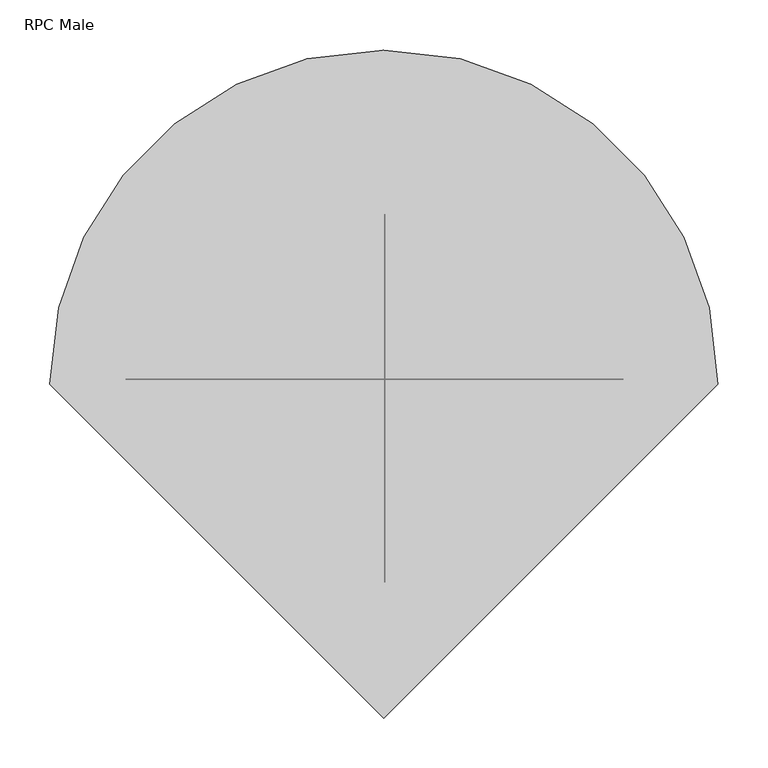
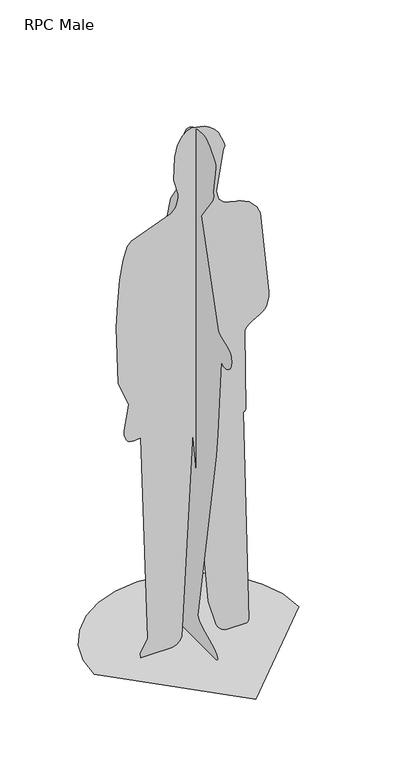
"""IFC4 building model written with IfcOpenShell, lengths in millimetres: proxy geometry, RPC Male : Dwayne."""

import ifcopenshell
import ifcopenshell.guid

model = None  # the IFC model being written
_history = None  # IfcOwnerHistory: only IFC2X3 demands one
_inside = {}  # id of a spatial element -> (the spatial element, [elements in it])
_under = {}  # id of a project, library or spatial element -> (it, [spatial elements below it])
_declared = {}  # id of a project -> (the project, [libraries it declares])
_typed = {}  # id of a type object -> (the type object, [elements of that type])
_made_of = {}  # id of a material, layer set ... -> (it, [elements and type objects made of it])


def new_model(schema):
    """Start an empty IFC model of exactly this schema.

    Asked for "IFC4X3", IfcOpenShell would pick the latest addendum, in which some entities
    have other attributes; the version numbers below select the first issue.
    IFC2X3 requires an IfcOwnerHistory on every rooted entity: one is made here for all.
    """
    global model, _history
    if schema == "IFC4X3":
        model = ifcopenshell.file(schema_version=(4, 3, 0, 0))
    else:
        model = ifcopenshell.file(schema=schema)
    _inside.clear()
    _under.clear()
    _declared.clear()
    _typed.clear()
    _made_of.clear()
    _history = None
    if model.schema == "IFC2X3":
        org = make("IfcOrganization", Name="unknown")
        user = make(
            "IfcPersonAndOrganization",
            ThePerson=make("IfcPerson", FamilyName="unknown"),
            TheOrganization=org,
        )
        app = make(
            "IfcApplication",
            ApplicationDeveloper=org,
            Version="unknown",
            ApplicationFullName="unknown",
            ApplicationIdentifier="unknown",
        )
        _history = make(
            "IfcOwnerHistory",
            OwningUser=user,
            OwningApplication=app,
            ChangeAction="ADDED",
            CreationDate=0,
        )
    return model


def make(cls, **values):
    """One entity of the class cls with the attributes given. An attribute that is None is left unset."""
    return model.create_entity(
        cls, **{name: value for name, value in values.items() if value is not None}
    )


def rooted(cls, **values):
    """An entity with a GlobalId (a new one), such as an element, a storey or a relation."""
    return make(cls, GlobalId=ifcopenshell.guid.new(), OwnerHistory=_history, **values)


def si_unit(unit_type, name, prefix=None):
    """IfcSIUnit, for example si_unit("LENGTHUNIT", "METRE", prefix="MILLI")."""
    return make("IfcSIUnit", UnitType=unit_type, Prefix=prefix, Name=name)


def assignment(units):
    """IfcUnitAssignment: the units of a project."""
    return None if units is None else make("IfcUnitAssignment", Units=units)


def point(xyz):
    """IfcCartesianPoint."""
    return None if xyz is None else make("IfcCartesianPoint", Coordinates=xyz)


def direction(xyz):
    """IfcDirection."""
    return None if xyz is None else make("IfcDirection", DirectionRatios=xyz)


def frame(location, z_axis=None, x_axis=None):
    """IfcAxis2Placement3D, a coordinate frame: its origin and axes. An axis left out is left unset."""
    return make(
        "IfcAxis2Placement3D",
        Location=point(location),
        Axis=direction(z_axis),
        RefDirection=direction(x_axis),
    )


def origin():
    """The frame at (0, 0, 0) with its axes left unset."""
    return frame((0.0, 0.0, 0.0))


def place(relative_to, where):
    """IfcLocalPlacement: puts the frame where relative to a parent placement (None: the world)."""
    return make(
        "IfcLocalPlacement", PlacementRelTo=relative_to, RelativePlacement=where
    )


def context(
    kind, dimensions, precision=None, world=None, true_north=None, identifier=None
):
    """IfcGeometricRepresentationContext, for example the 3D "Model" context."""
    return make(
        "IfcGeometricRepresentationContext",
        ContextIdentifier=identifier,
        ContextType=kind,
        CoordinateSpaceDimension=dimensions,
        Precision=precision,
        WorldCoordinateSystem=world,
        TrueNorth=true_north,
    )


def project(units=None, contexts=None):
    """IfcProject with its units and contexts."""
    return rooted(
        "IfcProject",
        Name="project",
        RepresentationContexts=contexts,
        UnitsInContext=assignment(units),
    )


def spatial(cls, under=None, at=None, **own):
    """A site, building, storey or space (cls), placed at a placement, below another one or the project."""
    s = rooted(cls, ObjectPlacement=at, **own)
    if under is not None:
        _under.setdefault(under.id(), (under, []))[1].append(s)
    return s


def point_list(points):
    """IfcCartesianPointList2D or 3D."""
    cls = (
        "IfcCartesianPointList2D" if len(points[0]) == 2 else "IfcCartesianPointList3D"
    )
    return make(cls, CoordList=points)


def triangles(points, corners, closed=None, point_numbers=None):
    """IfcTriangulatedFaceSet: each triangle names its three corners, points numbered from 1."""
    return make(
        "IfcTriangulatedFaceSet",
        Coordinates=point_list(points),
        Closed=closed,
        CoordIndex=corners,
        PnIndex=point_numbers,
    )


def shape(context_of_items, identifier, shape_type, items):
    """IfcShapeRepresentation: the items that make up one representation, for example the "Body"."""
    return make(
        "IfcShapeRepresentation",
        ContextOfItems=context_of_items,
        RepresentationIdentifier=identifier,
        RepresentationType=shape_type,
        Items=items,
    )


def source(mapping_origin, context_of_items, identifier, shape_type, items):
    """IfcRepresentationMap: a shape defined once, which mapped items show again and again."""
    return make(
        "IfcRepresentationMap",
        MappingOrigin=mapping_origin,
        MappedRepresentation=shape(context_of_items, identifier, shape_type, items),
    )


def transform(
    local_origin,
    x_axis=None,
    y_axis=None,
    z_axis=None,
    scale=None,
    scale2=None,
    scale3=None,
    uniform=True,
):
    """IfcCartesianTransformationOperator3D, or its non-uniform kind. x_axis, y_axis, z_axis: its Axis1, 2, 3."""
    if uniform:
        return make(
            "IfcCartesianTransformationOperator3D",
            Axis1=direction(x_axis),
            Axis2=direction(y_axis),
            LocalOrigin=point(local_origin),
            Scale=scale,
            Axis3=direction(z_axis),
        )
    return make(
        "IfcCartesianTransformationOperator3DnonUniform",
        Axis1=direction(x_axis),
        Axis2=direction(y_axis),
        LocalOrigin=point(local_origin),
        Scale=scale,
        Axis3=direction(z_axis),
        Scale2=scale2,
        Scale3=scale3,
    )


def mapped(mapping_source, mapping_target):
    """IfcMappedItem: shows the shape of a source again, moved by a transform."""
    return make(
        "IfcMappedItem", MappingSource=mapping_source, MappingTarget=mapping_target
    )


def made_of(thing, what):
    """Note that an element or type object is made of a material, layer set ...; save() writes the relation."""
    if what is not None:
        _made_of.setdefault(what.id(), (what, []))[1].append(thing)
    return thing


def element(
    cls,
    number,
    at=None,
    inside=None,
    cuts=None,
    type_object=None,
    material=None,
    context=None,
    identifier="Body",
    shape_type=None,
    held_by="IfcProductDefinitionShape",
    body=None,
    shapes=None,
    **own,
):
    """One element of the class cls, such as IfcWall. Its Tag is "e" and its number.

    at: its placement. inside: the storey or other place that contains it. cuts: it is an
    opening in that element (IfcRelVoidsElement). A single representation is given by context,
    identifier, shape_type and body (its items); several are given by shapes. held_by: the class
    of the entity that holds the representations. save() writes the other relations.
    """
    e = rooted(cls, Tag="e%d" % number, ObjectPlacement=at, **own)
    if body is not None:
        shapes = [shape(context, identifier, shape_type, body)]
    if shapes is not None:
        e.Representation = make(held_by, Representations=shapes)
    if inside is not None:
        _inside.setdefault(inside.id(), (inside, []))[1].append(e)
    if cuts is not None:
        rooted(
            "IfcRelVoidsElement", RelatingBuildingElement=cuts, RelatedOpeningElement=e
        )
    if type_object is not None:
        _typed.setdefault(type_object.id(), (type_object, []))[1].append(e)
    return made_of(e, material)


def aggregate(whole, parts):
    """IfcRelAggregates: a whole, such as a stair, and the parts it consists of."""
    return rooted("IfcRelAggregates", RelatingObject=whole, RelatedObjects=parts)


def save(model, path):
    """Write the relations noted so far, then the file.

    IfcRelAggregates (storeys below a building ...), IfcRelContainedInSpatialStructure (elements
    in a storey), IfcRelDefinesByType, IfcRelAssociatesMaterial and IfcRelDeclares: one each for
    every whole, place, type object, material and project.
    """
    for whole, parts in _under.values():
        aggregate(whole, parts)
    for where, things in _inside.values():
        rooted(
            "IfcRelContainedInSpatialStructure",
            RelatedElements=things,
            RelatingStructure=where,
        )
    for kind, things in _typed.values():
        rooted("IfcRelDefinesByType", RelatedObjects=things, RelatingType=kind)
    for what, things in _made_of.values():
        rooted("IfcRelAssociatesMaterial", RelatedObjects=things, RelatingMaterial=what)
    for by, libraries in _declared.values():
        rooted("IfcRelDeclares", RelatingContext=by, RelatedDefinitions=libraries)
    model.write(path)


def rpc_male_28878092(model_context):
    return source(origin(), model_context, "Body", "Tessellation", [
        triangles([(180.7519758, 4.45e-05, 5.61e-05), (184.2427693, 8.8e-06, 2.7953145), (186.1721755, -1.66e-05, 5.8375002), (186.8316374, -3.35e-05, 9.127569), (168.2846227, -8.5e-06, 733.0652109), (173.8813015, -8.5e-06, 735.2240908), (177.6698602, -8.1e-06, 740.93319), (174.1985423, 8.1e-06, 1013.6682867), (179.591309, 8.8e-06, 1024.1651751), (188.0395216, 9.6e-06, 1032.7759867), (198.5267085, 9.9e-06, 1040.1126028), (210.0363257, 1.03e-05, 1046.7864687), (221.5520472, 1.07e-05, 1053.4092476), (232.0572199, 1.1e-05, 1060.5929661), (240.5353907, 1.14e-05, 1068.9488514), (245.9518842, 1.21e-05, 1078.9880642), (249.7386988, 1.29e-05, 1091.9821838), (252.1552483, 1.4e-05, 1106.9298906), (253.4607645, 1.47e-05, 1122.8295742), (224.2188539, 3.16e-05, 1405.054644), (213.7949444, 3.31e-05, 1430.2019463), (189.1319694, 3.46e-05, 1456.0842327), (160.624934, 3.53e-05, 1468.8737137), (131.9229886, 3.57e-05, 1475.6378357), (106.6752928, 3.64e-05, 1483.4436092), (88.5310242, 3.71e-05, 1499.3593529), (81.1392697, 3.9e-05, 1530.4516411), (102.942045, 4.71e-05, 1666.4696468), (107.9472446, 4.78e-05, 1679.2650867), (108.1474504, 4.82e-05, 1680.5741638), (107.984815, 4.82e-05, 1682.7587688), (107.5268306, 4.82e-05, 1685.5190655), (106.840944, 4.86e-05, 1688.5553627), (86.6409052, 5.11e-05, 1733.0902897), (74.2774293, 5.19e-05, 1747.7183212), (59.5121605, 5.26e-05, 1759.6594528), (42.363121, 5.33e-05, 1768.7777916), (0.9855255, 5.37e-05, 1777.9990311), (-15.8808757, 5.33e-05, 1772.5528519), (-29.1619555, 5.26e-05, 1761.5639877), (-39.2640369, 5.19e-05, 1747.0962662), (-46.5934632, 5.08e-05, 1731.2140961), (-56.009163, 4.89e-05, 1695.7207684), (-59.1639487, 4.41e-05, 1618.2087845), (-44.4858339, 4.12e-05, 1564.7278919), (-44.3096682, 4.05e-05, 1551.1862766), (-46.5532813, 3.94e-05, 1537.9279289), (-51.2886345, 3.86e-05, 1525.4359589), (-58.5876575, 3.83e-05, 1514.1926044), (-68.5223164, 3.75e-05, 1504.6808304), (-198.4030241, 3.46e-05, 1454.5808361), (-210.7095586, 3.38e-05, 1440.8296406), (-224.9005892, 3.13e-05, 1397.8447643), (-235.5369131, 2.72e-05, 1333.6069702), (-242.7580384, 2.28e-05, 1256.1532677), (-246.7032373, 1.77e-05, 1173.5211021), (-240.2781571, 5.9e-06, 974.9290089), (-206.081389, 1.1e-06, 891.6222479), (-221.1961823, -4e-06, 805.6633232), (-220.4650678, -5.1e-06, 788.6200321), (-214.9948893, -6.3e-06, 771.8045614), (-210.3552016, -6.6e-06, 765.7300776), (-204.1668257, -6.6e-06, 762.0919275), (-196.8959759, -7e-06, 760.3982082), (-189.0090118, -7e-06, 760.1573799), (-180.9721295, -7e-06, 760.8774668), (-173.2515615, -6.6e-06, 762.0669291), (-166.3135766, -6.6e-06, 763.2339363), (-144.8011179, -4.49e-05, 59.4752896), (-168.6275342, -4.74e-05, 15.3365843), (-166.1985945, 4.45e-05, 5.61e-05), (-66.1332089, 4.45e-05, 5.61e-05), (-49.8425018, 1.03e-05, 3.9765591), (-39.0246256, -1.36e-05, 14.0353), (-32.5983009, -2.91e-05, 28.3297116), (2.7441046, -9.2e-06, 720.0458748), (54.0725034, -1.03e-05, 117.9433278), (81.3720135, 2.13e-05, 28.0047427), (85.5237041, 2.69e-05, 19.9172686), (91.2433859, 3.27e-05, 12.5691172), (99.2451413, 3.86e-05, 5.9378887), (110.2431982, 4.45e-05, 5.61e-05), (13.8237406, 127.6718764, 9.9621145), (13.8237974, 127.2617633, 182.0842528), (13.8237815, 135.2635732, 744.8695776), (13.8237815, 136.4149928, 748.3460369), (13.8237815, 139.3954704, 752.5736132), (13.8237815, 143.4944026, 757.5058702), (13.8237815, 148.0010861, 763.0962994), (13.8237815, 152.2049901, 769.2983917), (13.8237792, 155.3953659, 776.0656385), (13.8237792, 156.8616281, 783.3516764), (13.8237622, 165.9465024, 1358.6137287), (13.8237599, 143.2743216, 1442.0927902), (13.8237576, 71.1145501, 1552.8585583), (13.8237576, 64.3401725, 1580.5206779), (13.8237542, 73.5344014, 1684.7952724), (13.8237531, 67.2131212, 1712.2161278), (13.8237531, 55.241223, 1734.9070393), (13.8237531, 37.9260212, 1752.7537697), (13.8237531, 15.5748771, 1765.6426632), (13.8237531, -11.5049084, 1773.4593372), (13.8237531, -43.0059914, 1776.090136), (13.8237531, -55.0860226, 1772.9164925), (13.8237542, -79.7038559, 1756.3218658), (13.8237554, -107.4896145, 1722.3477768), (13.8237554, -111.5711695, 1713.01012), (13.8237554, -112.2229284, 1702.3019073), (13.8237588, -99.0832235, 1611.9284992), (13.8237588, -100.6007272, 1597.8206394), (13.8237599, -96.755177, 1579.0656796), (13.8237622, -31.1784566, 1488.4592915), (13.8237735, -125.7984261, 1146.7472277), (13.8237735, -134.1993577, 1137.675107), (13.8237747, -184.2799037, 1119.3925747), (13.8237747, -194.4649651, 1111.9394686), (13.8237747, -201.1343255, 1100.3801451), (13.8237769, -203.5508567, 1084.2058416), (13.8237769, -200.9674025, 1068.9640394), (13.8237769, -194.2820729, 1055.8707253), (13.8237769, -184.3928146, 1046.1415226), (13.8237769, -172.1978105, 1040.992709), (13.8237769, -158.595007, 1041.6399078), (13.8237769, -144.48246, 1049.299106), (13.8237838, -123.0429529, 785.7648285), (13.823786, -116.906318, 707.2429499), (13.8237928, -10.2023683, 90.6853168), (13.823794, -17.983895, 76.1481908), (13.8237951, -35.4714404, 63.806743), (13.8238042, -104.5965316, 31.8661463), (13.8238053, -119.3344402, 20.2173661), (13.8238076, -122.9915025, 6.7192091), (13.8238042, -122.0607091, 4.3674998), (13.8237894, -120.3451706, 2.3141478), (13.8237724, -119.1853577, 1.4285653), (13.8237474, -117.8199432, 0.6534771), (13.8237099, -116.2458387, 5.61e-05), (13.8237077, 124.501612, 0.0), (348.4734607, -4.7230039, 0.0001684), (339.5987117, 72.1961519, 0.0001684), (314.3237646, 142.8340959, 5.61e-05), (274.6722241, 205.1669827, 5.61e-05), (222.6681673, 257.171094, 5.61e-05), (160.3352533, 296.8225073, 5.61e-05), (89.6973139, 322.097527, 5.61e-05), (12.7781649, 330.972276, 5.61e-05), (-64.1409886, 322.0975634, 5.61e-05), (-134.7789371, 296.8225618, 5.61e-05), (-197.1118239, 257.1710577, 5.61e-05), (-249.1159897, 205.1670008, 5.61e-05), (-288.7673667, 142.8340595, 5.61e-05), (-314.0423864, 72.1960974, 0.0001684), (-322.9171354, -4.7230331, 0.0001684), (12.7782239, -340.4182474, 0.0001684)], [[70, 71, 72], [69, 70, 72], [69, 72, 73], [69, 73, 74], [69, 74, 75], [69, 75, 76], [68, 69, 76], [82, 1, 2], [82, 2, 3], [82, 3, 4], [81, 82, 4], [80, 81, 4], [79, 80, 4], [78, 79, 4], [77, 78, 4], [77, 4, 5], [76, 77, 5], [5, 6, 7], [76, 5, 7], [76, 7, 8], [68, 76, 8], [67, 68, 8], [66, 67, 8], [65, 66, 8], [64, 65, 8], [63, 64, 8], [62, 63, 8], [61, 62, 8], [60, 61, 8], [59, 60, 8], [58, 59, 8], [57, 58, 8], [56, 57, 8], [56, 8, 9], [55, 56, 9], [55, 9, 10], [54, 55, 10], [54, 10, 11], [53, 54, 11], [53, 11, 12], [52, 53, 12], [51, 52, 12], [50, 51, 12], [50, 12, 13], [50, 13, 14], [50, 14, 15], [50, 15, 16], [50, 16, 17], [50, 17, 18], [50, 18, 19], [50, 19, 20], [50, 20, 21], [50, 21, 22], [50, 22, 23], [50, 23, 24], [50, 24, 25], [50, 25, 26], [49, 50, 26], [48, 49, 26], [48, 26, 27], [47, 48, 27], [46, 47, 27], [45, 46, 27], [44, 45, 27], [44, 27, 28], [43, 44, 28], [42, 43, 28], [42, 28, 29], [42, 29, 30], [42, 30, 31], [42, 31, 32], [42, 32, 33], [42, 33, 34], [42, 34, 35], [42, 35, 36], [42, 36, 37], [41, 42, 37], [40, 41, 37], [40, 37, 38], [40, 38, 39], [137, 138, 83], [137, 83, 84], [136, 137, 84], [135, 136, 84], [130, 131, 132], [130, 132, 133], [130, 133, 134], [130, 134, 135], [122, 123, 124], [121, 122, 124], [120, 121, 124], [119, 120, 124], [118, 119, 124], [117, 118, 124], [116, 117, 124], [115, 116, 124], [114, 115, 124], [113, 114, 124], [106, 107, 108], [105, 106, 108], [104, 105, 108], [103, 104, 108], [102, 103, 108], [101, 102, 108], [100, 101, 108], [99, 100, 108], [98, 99, 108], [97, 98, 108], [97, 108, 109], [97, 109, 110], [97, 110, 111], [96, 97, 111], [95, 96, 111], [95, 111, 112], [94, 95, 112], [93, 94, 112], [93, 112, 113], [92, 93, 113], [92, 113, 124], [92, 124, 125], [91, 92, 125], [90, 91, 125], [89, 90, 125], [88, 89, 125], [87, 88, 125], [86, 87, 125], [86, 125, 126], [85, 86, 126], [85, 126, 127], [84, 85, 127], [84, 127, 128], [135, 84, 128], [135, 128, 129], [130, 135, 129], [153, 154, 139], [152, 153, 139], [152, 139, 140], [151, 152, 140], [151, 140, 141], [151, 141, 142], [150, 151, 142], [149, 150, 142], [149, 142, 143], [149, 143, 144], [149, 144, 145], [149, 145, 146], [149, 146, 147], [149, 147, 148]], closed=False),
    ])


if __name__ == "__main__":
    model = new_model("IFC4")
    model_context = context("Model", 3, world=origin())
    ifc_project = project(units=[si_unit("LENGTHUNIT", "METRE", prefix="MILLI")], contexts=[model_context])
    site = spatial("IfcSite", under=ifc_project)
    building = spatial("IfcBuilding", under=site)
    placement = place(None, origin())
    rpc_male_shape = rpc_male_28878092(model_context)
    element("IfcBuildingElementProxy", 1, Name="RPC Male : Dwayne", ObjectType="RPC Male : Dwayne", at=placement, inside=building, context=model_context, shape_type="MappedRepresentation", body=[
        mapped(rpc_male_shape, transform((0.0, 0.0, 0.0), x_axis=(1.0, 0.0, 0.0), y_axis=(0.0, 1.0, 0.0), z_axis=(0.0, 0.0, 1.0))),
    ])
    save(model, "model.ifc")

# Revit data of these elements
# Type "RPC Male : Dwayne"
#   built-in parameter 1005198 = "{2, 15},{22, RPC-8-G1AE-S4G0-CKUK-A},{1, 0},{1, 0},{2, 15},{1, 8},{5, Color},{1, 0},{1, 0},{3, 0.8},{3, 0.8},{3, 0.8},{1, 8},{7, BBoxMin},{1, 0},{1, 0},{1, 0},{1, 0},{1, 0},{1, 8},{7, BBoxMax},{1, 0},{1, 0},{1, 0},{1, 0},{1, 0},{2, 11},{9, RPCTypeId},{1, 0},{1, 0},{22, RPC-8-G1AE-S4G0-CKUK-A},{1, 6},{14, RPCPlantHeight},{1, 0},{1, 0},{7, 5.83333},{2, 11},{7, keyword},{1, 0},{1, 0},{45, :RPCs:People [Business-Hispanic]:Geometry:RPC},{2, 11},{8, category},{1, 0},{1, 0},{26, People [Business-Hispanic]},{2, 11},{12, LocalizedUID},{1, 0},{1, 0},{6, Dwayne},{2, 14},{6, Height},{1, 0},{1, 0},{7, 5.83333},{1, 2},{16, Cast Reflections},{1, 0},{1, 0},{1, 0},{1, 2},{6, Jitter},{1, 0},{1, 0},{1, 1},{1, 2},{9, Billboard},{1, 0},{1, 0},{1, 0},{1, 2},{12, Cast Shadows},{1, 0},{1, 0},{1, 1},{1, 2},{20, Apply Filter Effects},{1, 0},{1, 0},{1, 0},{2, 11},{28, Apply Filter Effects-Text-FC},{1, 0},{1, 0},{4, None},{21, assetlibrary_base.fbx},{1, 5},"
#   built-in parameter 1005195 = "RPC-8-G1AE-S4G0-CKUK-A"
#   Height = 0
